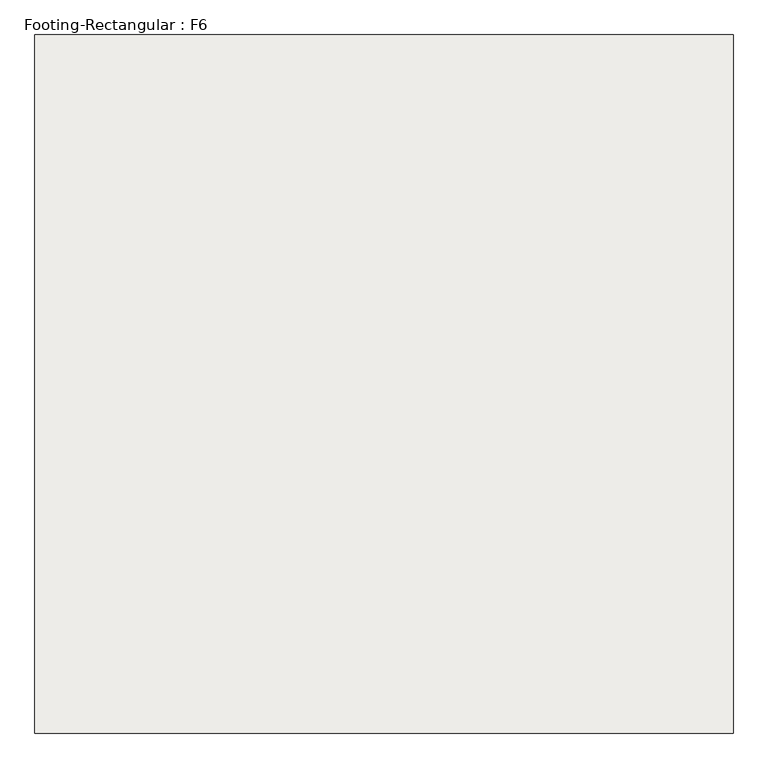
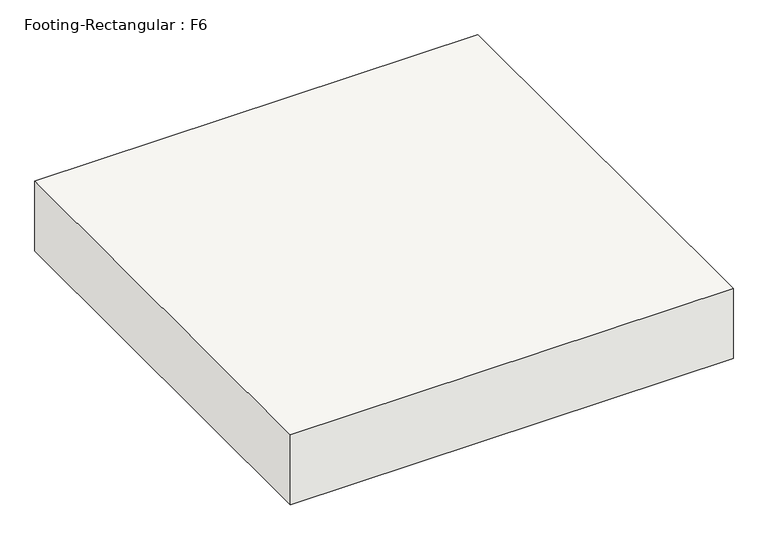
"""IFC4 building model written with IfcOpenShell, lengths in millimetres: slab geometry, Footing-Rectangular : F6."""

from ifc_helpers import new_model, si_unit, frame, origin, place, context, project, spatial, polyline, outline, extrude, source, transform, mapped, element, save


def footing_rectangular_f6_e8c3e57f(model_context):
    return source(origin(), model_context, "Body", "SweptSolid", [
        extrude(outline(polyline([(914.4, 914.4), (914.4, -914.4), (-914.4, -914.4), (-914.4, 914.4), (914.4, 914.4)])), frame((0.0, 0.0, -304.8), z_axis=(0.0, 0.0, 1.0), x_axis=(1.0, 0.0, 0.0)), (0.0, 0.0, 1.0), 304.8),
    ])


if __name__ == "__main__":
    model = new_model("IFC4")
    model_context = context("Model", 3, world=origin())
    ifc_project = project(units=[si_unit("LENGTHUNIT", "METRE", prefix="MILLI")], contexts=[model_context])
    site = spatial("IfcSite", under=ifc_project)
    building = spatial("IfcBuilding", under=site)
    placement = place(None, origin())
    footing_rectangular_f6_shape = footing_rectangular_f6_e8c3e57f(model_context)
    element("IfcSlab", 1, ObjectType="Footing-Rectangular : F6", at=placement, inside=building, context=model_context, shape_type="MappedRepresentation", body=[
        mapped(footing_rectangular_f6_shape, transform((0.0, 0.0, 0.0), x_axis=(1.0, 0.0, 0.0), y_axis=(0.0, 1.0, 0.0), z_axis=(0.0, 0.0, 1.0))),
    ])
    save(model, "model.ifc")

# Revit data of these elements
# Type "Footing-Rectangular : F6"
#   Assembly Code = "A1010100"
#   Width = 6' - 0"
#   Length = 6' - 0"
#   Foundation Thickness = 1' - 0"
#   Structural Material [instance default] = Concrete, Cast-in-Place gray
# Element 1 (IfcSlab, "Footing-Rectangular : F6")
#   Materials on its faces: "Concrete, Cast-in-Place gray"
# Materials
#   "Concrete, Cast-in-Place gray": class "Concrete", colour RGB 192 192 192, transparency 0, Description = "Cast-in-place concrete", Cost = 0
